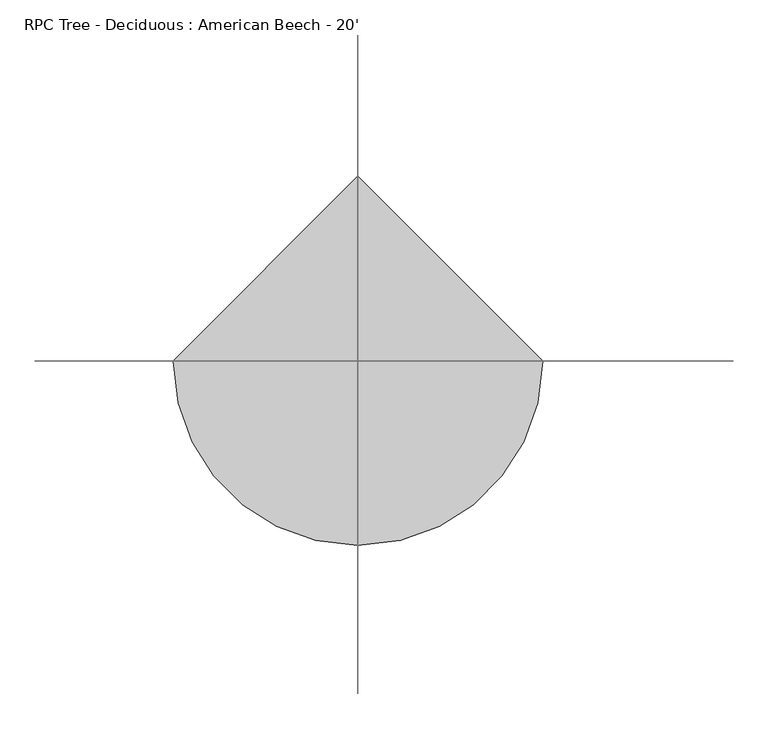
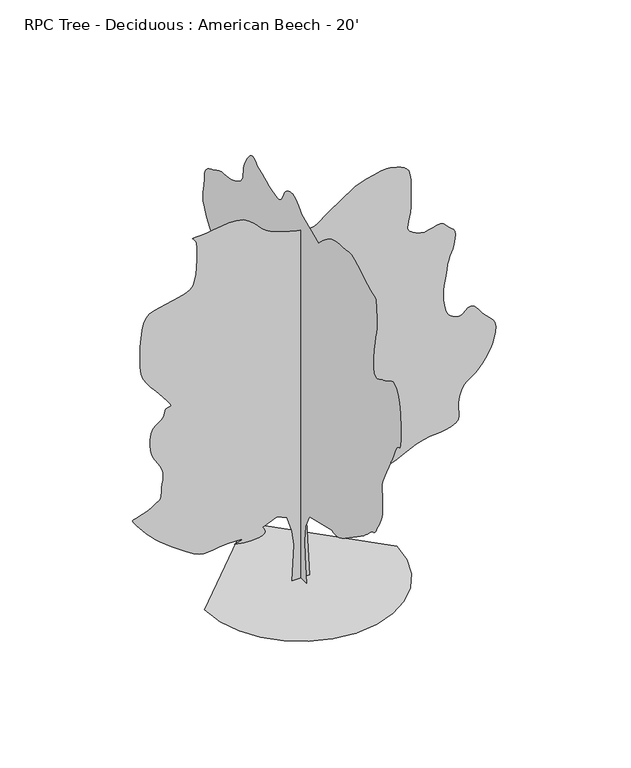
"""IFC4 building model written with IfcOpenShell, lengths in millimetres: geographic element geometry, RPC Tree - Deciduous : American Beech - 20'."""

import ifcopenshell
import ifcopenshell.guid

model = None  # the IFC model being written
_history = None  # IfcOwnerHistory: only IFC2X3 demands one
_inside = {}  # id of a spatial element -> (the spatial element, [elements in it])
_under = {}  # id of a project, library or spatial element -> (it, [spatial elements below it])
_declared = {}  # id of a project -> (the project, [libraries it declares])
_typed = {}  # id of a type object -> (the type object, [elements of that type])
_made_of = {}  # id of a material, layer set ... -> (it, [elements and type objects made of it])


def new_model(schema):
    """Start an empty IFC model of exactly this schema.

    Asked for "IFC4X3", IfcOpenShell would pick the latest addendum, in which some entities
    have other attributes; the version numbers below select the first issue.
    IFC2X3 requires an IfcOwnerHistory on every rooted entity: one is made here for all.
    """
    global model, _history
    if schema == "IFC4X3":
        model = ifcopenshell.file(schema_version=(4, 3, 0, 0))
    else:
        model = ifcopenshell.file(schema=schema)
    _inside.clear()
    _under.clear()
    _declared.clear()
    _typed.clear()
    _made_of.clear()
    _history = None
    if model.schema == "IFC2X3":
        org = make("IfcOrganization", Name="unknown")
        user = make(
            "IfcPersonAndOrganization",
            ThePerson=make("IfcPerson", FamilyName="unknown"),
            TheOrganization=org,
        )
        app = make(
            "IfcApplication",
            ApplicationDeveloper=org,
            Version="unknown",
            ApplicationFullName="unknown",
            ApplicationIdentifier="unknown",
        )
        _history = make(
            "IfcOwnerHistory",
            OwningUser=user,
            OwningApplication=app,
            ChangeAction="ADDED",
            CreationDate=0,
        )
    return model


def make(cls, **values):
    """One entity of the class cls with the attributes given. An attribute that is None is left unset."""
    return model.create_entity(
        cls, **{name: value for name, value in values.items() if value is not None}
    )


def rooted(cls, **values):
    """An entity with a GlobalId (a new one), such as an element, a storey or a relation."""
    return make(cls, GlobalId=ifcopenshell.guid.new(), OwnerHistory=_history, **values)


def si_unit(unit_type, name, prefix=None):
    """IfcSIUnit, for example si_unit("LENGTHUNIT", "METRE", prefix="MILLI")."""
    return make("IfcSIUnit", UnitType=unit_type, Prefix=prefix, Name=name)


def assignment(units):
    """IfcUnitAssignment: the units of a project."""
    return None if units is None else make("IfcUnitAssignment", Units=units)


def point(xyz):
    """IfcCartesianPoint."""
    return None if xyz is None else make("IfcCartesianPoint", Coordinates=xyz)


def direction(xyz):
    """IfcDirection."""
    return None if xyz is None else make("IfcDirection", DirectionRatios=xyz)


def frame(location, z_axis=None, x_axis=None):
    """IfcAxis2Placement3D, a coordinate frame: its origin and axes. An axis left out is left unset."""
    return make(
        "IfcAxis2Placement3D",
        Location=point(location),
        Axis=direction(z_axis),
        RefDirection=direction(x_axis),
    )


def origin():
    """The frame at (0, 0, 0) with its axes left unset."""
    return frame((0.0, 0.0, 0.0))


def place(relative_to, where):
    """IfcLocalPlacement: puts the frame where relative to a parent placement (None: the world)."""
    return make(
        "IfcLocalPlacement", PlacementRelTo=relative_to, RelativePlacement=where
    )


def context(
    kind, dimensions, precision=None, world=None, true_north=None, identifier=None
):
    """IfcGeometricRepresentationContext, for example the 3D "Model" context."""
    return make(
        "IfcGeometricRepresentationContext",
        ContextIdentifier=identifier,
        ContextType=kind,
        CoordinateSpaceDimension=dimensions,
        Precision=precision,
        WorldCoordinateSystem=world,
        TrueNorth=true_north,
    )


def project(units=None, contexts=None):
    """IfcProject with its units and contexts."""
    return rooted(
        "IfcProject",
        Name="project",
        RepresentationContexts=contexts,
        UnitsInContext=assignment(units),
    )


def spatial(cls, under=None, at=None, **own):
    """A site, building, storey or space (cls), placed at a placement, below another one or the project."""
    s = rooted(cls, ObjectPlacement=at, **own)
    if under is not None:
        _under.setdefault(under.id(), (under, []))[1].append(s)
    return s


def point_list(points):
    """IfcCartesianPointList2D or 3D."""
    cls = (
        "IfcCartesianPointList2D" if len(points[0]) == 2 else "IfcCartesianPointList3D"
    )
    return make(cls, CoordList=points)


def triangles(points, corners, closed=None, point_numbers=None):
    """IfcTriangulatedFaceSet: each triangle names its three corners, points numbered from 1."""
    return make(
        "IfcTriangulatedFaceSet",
        Coordinates=point_list(points),
        Closed=closed,
        CoordIndex=corners,
        PnIndex=point_numbers,
    )


def shape(context_of_items, identifier, shape_type, items):
    """IfcShapeRepresentation: the items that make up one representation, for example the "Body"."""
    return make(
        "IfcShapeRepresentation",
        ContextOfItems=context_of_items,
        RepresentationIdentifier=identifier,
        RepresentationType=shape_type,
        Items=items,
    )


def source(mapping_origin, context_of_items, identifier, shape_type, items):
    """IfcRepresentationMap: a shape defined once, which mapped items show again and again."""
    return make(
        "IfcRepresentationMap",
        MappingOrigin=mapping_origin,
        MappedRepresentation=shape(context_of_items, identifier, shape_type, items),
    )


def transform(
    local_origin,
    x_axis=None,
    y_axis=None,
    z_axis=None,
    scale=None,
    scale2=None,
    scale3=None,
    uniform=True,
):
    """IfcCartesianTransformationOperator3D, or its non-uniform kind. x_axis, y_axis, z_axis: its Axis1, 2, 3."""
    if uniform:
        return make(
            "IfcCartesianTransformationOperator3D",
            Axis1=direction(x_axis),
            Axis2=direction(y_axis),
            LocalOrigin=point(local_origin),
            Scale=scale,
            Axis3=direction(z_axis),
        )
    return make(
        "IfcCartesianTransformationOperator3DnonUniform",
        Axis1=direction(x_axis),
        Axis2=direction(y_axis),
        LocalOrigin=point(local_origin),
        Scale=scale,
        Axis3=direction(z_axis),
        Scale2=scale2,
        Scale3=scale3,
    )


def mapped(mapping_source, mapping_target):
    """IfcMappedItem: shows the shape of a source again, moved by a transform."""
    return make(
        "IfcMappedItem", MappingSource=mapping_source, MappingTarget=mapping_target
    )


def made_of(thing, what):
    """Note that an element or type object is made of a material, layer set ...; save() writes the relation."""
    if what is not None:
        _made_of.setdefault(what.id(), (what, []))[1].append(thing)
    return thing


def element(
    cls,
    number,
    at=None,
    inside=None,
    cuts=None,
    type_object=None,
    material=None,
    context=None,
    identifier="Body",
    shape_type=None,
    held_by="IfcProductDefinitionShape",
    body=None,
    shapes=None,
    **own,
):
    """One element of the class cls, such as IfcWall. Its Tag is "e" and its number.

    at: its placement. inside: the storey or other place that contains it. cuts: it is an
    opening in that element (IfcRelVoidsElement). A single representation is given by context,
    identifier, shape_type and body (its items); several are given by shapes. held_by: the class
    of the entity that holds the representations. save() writes the other relations.
    """
    e = rooted(cls, Tag="e%d" % number, ObjectPlacement=at, **own)
    if body is not None:
        shapes = [shape(context, identifier, shape_type, body)]
    if shapes is not None:
        e.Representation = make(held_by, Representations=shapes)
    if inside is not None:
        _inside.setdefault(inside.id(), (inside, []))[1].append(e)
    if cuts is not None:
        rooted(
            "IfcRelVoidsElement", RelatingBuildingElement=cuts, RelatedOpeningElement=e
        )
    if type_object is not None:
        _typed.setdefault(type_object.id(), (type_object, []))[1].append(e)
    return made_of(e, material)


def aggregate(whole, parts):
    """IfcRelAggregates: a whole, such as a stair, and the parts it consists of."""
    return rooted("IfcRelAggregates", RelatingObject=whole, RelatedObjects=parts)


def save(model, path):
    """Write the relations noted so far, then the file.

    IfcRelAggregates (storeys below a building ...), IfcRelContainedInSpatialStructure (elements
    in a storey), IfcRelDefinesByType, IfcRelAssociatesMaterial and IfcRelDeclares: one each for
    every whole, place, type object, material and project.
    """
    for whole, parts in _under.values():
        aggregate(whole, parts)
    for where, things in _inside.values():
        rooted(
            "IfcRelContainedInSpatialStructure",
            RelatedElements=things,
            RelatingStructure=where,
        )
    for kind, things in _typed.values():
        rooted("IfcRelDefinesByType", RelatedObjects=things, RelatingType=kind)
    for what, things in _made_of.values():
        rooted("IfcRelAssociatesMaterial", RelatedObjects=things, RelatingMaterial=what)
    for by, libraries in _declared.values():
        rooted("IfcRelDeclares", RelatingContext=by, RelatedDefinitions=libraries)
    model.write(path)


def rpc_tree_deciduous_american_beech_20_b3c041c8(model_context):
    return source(origin(), model_context, "Body", "Tessellation", [
        triangles([(0.0009889, 136.856581, 0.0), (0.0009889, -149.8547884, 0.0), (0.0009889, -111.6264895, 420.510052), (0.0009889, -102.0697236, 659.4353302), (0.0009889, -121.1832463, 898.3606447), (0.0009889, -235.8678885, 1118.172373), (0.0009889, -818.8458761, 1261.5275036), (0.0009889, -849.9431059, 1249.7139805), (0.0009889, -883.2933231, 1240.7427258), (0.0009889, -921.1596891, 1237.4533916), (0.0009889, -965.7976622, 1242.6934788), (0.0009889, -1019.4603024, 1259.3000233), (0.0009889, -1084.4081549, 1290.1152935), (0.0009889, -1162.8992941, 1337.984174), (0.0009889, -1478.2811337, 1557.7959023), (0.0009889, -1522.8632961, 1589.1420994), (0.0009889, -1566.942437, 1618.9819931), (0.0009889, -1611.1893002, 1649.3249084), (0.0009889, -1656.2718681, 1682.1772636), (0.0009889, -1702.8579781, 1719.5406807), (0.0009889, -1751.6183739, 1763.4243393), (0.0009889, -1803.2210381, 1815.834803), (0.0009889, -1847.9404015, 1858.0191467), (0.0009889, -1878.9512993, 1877.1351311), (0.0009889, -1901.2702858, 1884.0440117), (0.0009889, -1919.9112991, 1889.616782), (0.0009889, -1939.8884228, 1904.7196392), (0.0009889, -1966.2180656, 1940.2161644), (0.0009889, -2003.916782, 2006.9774963), (0.0009889, -2044.9607883, 2083.2080177), (0.0009889, -2078.313549, 2145.2324295), (0.0009889, -2104.4754696, 2201.0692829), (0.0009889, -2123.9521877, 2258.7475937), (0.0009889, -2137.244109, 2326.2862038), (0.0009889, -2144.8488773, 2411.7141289), (0.0009889, -2147.2746014, 2523.0550072), (0.0009889, -2142.5373905, 2624.8889076), (0.0009889, -2132.7863869, 2688.2873634), (0.0009889, -2124.7040314, 2730.9338882), (0.0009889, -2124.9835201, 2770.583503), (0.0009889, -2140.3072941, 2824.9394875), (0.0009889, -2177.3659332, 2911.7568626), (0.0009889, -2242.84464, 3048.6883301), (0.0009889, -2308.7119858, 3181.9621719), (0.0009889, -2348.5011269, 3259.3812836), (0.0009889, -2371.2366577, 3301.215358), (0.0009889, -2385.9484051, 3327.6567673), (0.0009889, -2401.6632889, 3358.9496246), (0.0009889, -2427.4088104, 3415.3121727), (0.0009889, -2472.2118896, 3516.9885246), (0.0009889, -2522.8114174, 3609.6476944), (0.0009889, -2561.0332123, 3645.1568642), (0.0009889, -2588.5669968, 3652.9040657), (0.0009889, -2607.0580193, 3662.3273277), (0.0009889, -2618.2087921, 3702.8402618), (0.0009889, -2623.669796, 3803.856189), (0.0009889, -2625.117382, 3994.8390083), (0.0009889, -2615.3639076, 4210.713913), (0.0009889, -2589.2271309, 4371.4450905), (0.0009889, -2551.406765, 4483.8402649), (0.0009889, -2506.5400269, 4554.7824463), (0.0009889, -2459.3391289, 4591.1043571), (0.0009889, -2414.4802391, 4599.6895889), (0.0009889, -2376.641851, 4587.3705734), (0.0009889, -2343.8477772, 4566.9491455), (0.0009889, -2310.8862717, 4546.8576393), (0.0009889, -2277.5893215, 4527.4521378), (0.0009889, -2243.7921112, 4509.0116936), (0.0009889, -2209.3243023, 4491.9426773), (0.0009889, -2174.0232594, 4476.5250137), (0.0009889, -2137.7164639, 4463.1392029), (0.0009889, -2096.4236355, 4443.6572525), (0.0009889, -2049.6139927, 4418.4858238), (0.0009889, -2002.3013283, 4400.6805153), (0.0009889, -1959.504958, 4403.2713455), (0.0009889, -1926.2359131, 4439.313913), (0.0009889, -1907.5110386, 4521.8132378), (0.0009889, -1908.3467434, 4663.8246277), (0.0009889, -1923.6450829, 4819.4253044), (0.0009889, -1942.954224, 4940.7356323), (0.0009889, -1963.266647, 5037.9669067), (0.0009889, -1981.572361, 5121.3298416), (0.0009889, -1994.8642822, 5201.0354416), (0.0009889, -2000.1296585, 5287.2429703), (0.0009889, -1994.3614059, 5390.1634323), (0.0009889, -1986.3653824, 5488.9190323), (0.0009889, -1983.048143, 5559.911792), (0.0009889, -1978.5625156, 5609.3407516), (0.0009889, -1967.0562412, 5643.3764648), (0.0009889, -1942.6748806, 5668.2429703), (0.0009889, -1899.5709709, 5690.0869858), (0.0009889, -1831.8926891, 5715.1063889), (0.0009889, -1748.4408062, 5751.9616974), (0.0009889, -1662.820015, 5800.5261749), (0.0009889, -1576.3582867, 5853.7903656), (0.0009889, -1490.4020508, 5904.6919098), (0.0009889, -1406.2848015, 5946.2207703), (0.0009889, -1325.3426491, 5971.3924896), (0.0009889, -1248.913884, 5973.1447083), (0.0009889, -1174.2403896, 5963.3406555), (0.0009889, -1098.5636135, 5956.711409), (0.0009889, -1023.222064, 5950.5641098), (0.0009889, -949.5518515, 5942.2588028), (0.0009889, -878.8914843, 5929.1264648), (0.0009889, -812.5771454, 5908.4509827), (0.0009889, -751.9472706, 5877.5644958), (0.0009889, -697.9494038, 5841.2678741), (0.0009889, -649.9687569, 5805.9618896), (0.0009889, -607.0045916, 5771.4942261), (0.0009889, -568.0511189, 5737.7119858), (0.0009889, -532.1075644, 5704.4128555), (0.0009889, -498.1706097, 5671.4433563), (0.0009889, -465.2369368, 5638.6523346), (0.0009889, -16.056217, 5829.7871796), (0.0009889, 22.8405617, 5872.4339951), (0.0009889, 61.6537222, 5913.023378), (0.0009889, 100.2998553, 5949.3961578), (0.0009889, 138.6950317, 5979.5204819), (0.0009889, 176.7559443, 6001.2883392), (0.0009889, 214.3990318, 6012.5911377), (0.0009889, 251.5404602, 6011.3720261), (0.0009889, 287.2056524, 6002.4312927), (0.0009889, 320.3628219, 5991.305809), (0.0009889, 350.8454089, 5977.0055191), (0.0009889, 378.4856913, 5958.5397858), (0.0009889, 403.1160919, 5934.892392), (0.0009889, 424.5689612, 5905.047702), (0.0009889, 442.6817001, 5868.0144974), (0.0009889, 459.9562634, 5826.9425858), (0.0009889, 480.2407084, 5787.547316), (0.0009889, 505.3740581, 5752.6727005), (0.0009889, 537.1926464, 5725.138916), (0.0009889, 577.5380399, 5707.7911377), (0.0009889, 628.2491524, 5703.5239563), (0.0009889, 691.1650068, 5715.1063889), (0.0009889, 759.6790661, 5736.9754028), (0.0009889, 826.1890326, 5761.3593796), (0.0009889, 891.0251186, 5787.8263687), (0.0009889, 954.5251671, 5815.9694183), (0.0009889, 1017.0218611, 5845.3577408), (0.0009889, 1078.8506453, 5875.5832214), (0.0009889, 1140.3440575, 5906.2412338), (0.0009889, 1169.0715191, 5932.3524307), (0.0009889, 1198.1316639, 5955.3649796), (0.0009889, 1227.8624073, 5972.2052307), (0.0009889, 1258.5938164, 5979.7489563), (0.0009889, 1290.6664227, 5974.9230881), (0.0009889, 1324.4078224, 5954.6539764), (0.0009889, 1360.1557858, 5915.7918137), (0.0009889, 1395.1799561, 5868.217392), (0.0009889, 1426.1908539, 5822.9544571), (0.0009889, 1452.6880737, 5778.8856354), (0.0009889, 1474.1715008, 5734.7912338), (0.0009889, 1490.1379681, 5689.5538788), (0.0009889, 1500.0845993, 5641.9538773), (0.0009889, 1503.510989, 5590.8494385), (0.0009889, 1507.2168674, 5539.3380478), (0.0009889, 1519.1142517, 5491.1793594), (0.0009889, 1540.3740005, 5446.1704788), (0.0009889, 1572.1672634, 5404.1846695), (0.0009889, 1615.6596668, 5365.0428726), (0.0009889, 1672.0274471, 5328.5689362), (0.0009889, 1742.4363762, 5294.5832199), (0.0009889, 1817.5288857, 5269.1836075), (0.0009889, 1887.9378147, 5255.1373718), (0.0009889, 1954.8363476, 5247.4407486), (0.0009889, 2019.3956337, 5241.0911362), (0.0009889, 2082.7839157, 5231.0580276), (0.0009889, 2146.1721977, 5212.3382401), (0.0009889, 2210.7313385, 5179.9024292), (0.0009889, 2276.3498623, 5145.3580261), (0.0009889, 2340.1267834, 5118.8404587), (0.0009889, 2399.0573433, 5093.1356323), (0.0009889, 2450.1315514, 5061.106192), (0.0009889, 2490.3372368, 5015.5136261), (0.0009889, 2516.667025, 4949.193837), (0.0009889, 2526.1132507, 4854.9597633), (0.0009889, 2532.46577, 4758.008123), (0.0009889, 2546.5044479, 4681.9348595), (0.0009889, 2560.7285797, 4617.2411339), (0.0009889, 2567.5865913, 4554.3760757), (0.0009889, 2559.5600464, 4483.8402649), (0.0009889, 2529.1232414, 4396.0578323), (0.0009889, 2468.7702393, 4281.5543564), (0.0009889, 2394.0992157, 4166.6192207), (0.0009889, 2326.6139454, 4078.2525215), (0.0009889, 2267.6553349, 4007.9707649), (0.0009889, 2218.5596397, 3947.1884285), (0.0009889, 2180.6679119, 3887.4223091), (0.0009889, 2155.3111748, 3820.1377533), (0.0009889, 2143.8328056, 3736.8001076), (0.0009889, 2149.4334812, 3646.0204742), (0.0009889, 2171.0820145, 3561.7686401), (0.0009889, 2203.7667927, 3483.5112076), (0.0009889, 2242.4687908, 3410.790937), (0.0009889, 2282.1714546, 3343.1000107), (0.0009889, 2317.8662235, 3279.9047401), (0.0009889, 2344.5311657, 3220.7225967), (0.0009889, 2370.3577869, 3180.6921913), (0.0009889, 2402.5396889, 3164.8934464), (0.0009889, 2434.5538685, 3157.7813805), (0.0009889, 2459.8827003, 3143.8113029), (0.0009889, 2472.0037628, 3107.4638123), (0.0009889, 2464.3963783, 3033.1433487), (0.0009889, 2430.5432121, 2905.3305107), (0.0009889, 2383.9011463, 2761.3378464), (0.0009889, 2340.6017544, 2643.9136185), (0.0009889, 2298.1379219, 2545.7425758), (0.0009889, 2254.0028252, 2459.415287), (0.0009889, 2205.6894951, 2377.6095245), (0.0009889, 2150.6857304, 2292.9614937), (0.0009889, 2086.4897942, 2198.1177189), (0.0009889, 2022.098085, 2102.5196297), (0.0009889, 1968.0723129, 2019.6267242), (0.0009889, 1924.2446102, 1948.102747), (0.0009889, 1890.4447838, 1886.6067913), (0.0009889, 1866.5103436, 1833.8078339), (0.0009889, 1852.2735672, 1788.3620613), (0.0009889, 1847.564407, 1748.9361248), (0.0009889, 1851.5776794, 1721.8800728), (0.0009889, 1860.940044, 1709.2029396), (0.0009889, 1871.6386642, 1703.0459026), (0.0009889, 1879.6624477, 1695.5504299), (0.0009889, 1881.0010288, 1678.8600243), (0.0009889, 1871.6386642, 1645.1186245), (0.0009889, 1847.564407, 1586.4675533), (0.0009889, 1827.5314728, 1524.5828133), (0.0009889, 1825.3850922, 1482.2587978), (0.0009889, 1829.7590984, 1453.3104195), (0.0009889, 1829.2865982, 1431.547649), (0.0009889, 1812.5961926, 1410.7907764), (0.0009889, 1768.3214241, 1384.8497726), (0.0009889, 1685.0958355, 1347.5421661), (0.0009889, 1594.399918, 1309.4244347), (0.0009889, 1528.281134, 1282.5080544), (0.0009889, 1476.2059696, 1262.7823689), (0.0009889, 1427.6412014, 1246.2316349), (0.0009889, 1372.05317, 1228.8453415), (0.0009889, 1298.9138844, 1206.6102161), (0.0009889, 1197.6871416, 1175.5154572), (0.0009889, 1096.069289, 1145.7009253), (0.0009889, 1022.5387482, 1127.7557997), (0.0009889, 967.7331545, 1118.3400227), (0.0009889, 922.2874546, 1114.10329), (0.0009889, 876.8442255, 1111.7080873), (0.0009889, 822.0360884, 1107.806654), (0.0009889, 748.5055475, 1099.0588594), (0.0009889, 662.4935011, 1085.0990284), (0.0009889, 576.4788749, 1068.1292793), (0.0009889, 490.4667558, 1048.6551046), (0.0009889, 404.4521296, 1027.1717503), (0.0009889, 318.4400468, 1004.1847086), (0.0009889, 232.4266923, 980.1943851), (0.0009889, 146.4133378, 955.7037289), (136.1842383, 0.0003154, 0.014068), (-131.4120823, 0.0003154, 0.014068), (-102.7410489, 0.0002819, 563.8778998), (-131.4120823, 0.0002692, 793.2477293), (-207.8684348, 0.0002549, 1032.1729712), (-360.7819027, 0.0002501, 1108.6296415), (-580.5936673, 0.0002549, 1013.0594576), (-562.704425, 0.0002564, 988.5662579), (-548.0765751, 0.000258, 964.5784779), (-539.9688578, 0.0002596, 941.5914362), (-541.6401947, 0.0002612, 920.1080818), (-556.3518694, 0.0002628, 900.6313637), (-587.3627672, 0.0002628, 883.6641581), (-637.9342443, 0.0002644, 869.704327), (-697.421093, 0.0002644, 860.4815615), (-753.4001616, 0.0002644, 856.775683), (-806.4506298, 0.0002644, 857.667271), (-857.1617786, 0.0002644, 862.2366869), (-906.117802, 0.0002644, 869.5645826), (-953.9028214, 0.0002628, 878.731465), (-1001.1011759, 0.0002628, 888.8178406), (-953.2881786, 0.0002628, 900.9945683), (-913.501581, 0.0002612, 912.5008427), (-889.7601522, 0.0002612, 922.6710068), (-890.0954515, 0.0002596, 930.8345346), (-922.5287189, 0.0002596, 936.3235165), (-995.0838833, 0.0002596, 938.4698244), (-1115.7848007, 0.0002596, 936.6028599), (-1242.9524746, 0.0002612, 927.8271601), (-1337.3542706, 0.0002612, 914.3677345), (-1410.6891838, 0.0002612, 903.2500992), (-1474.6617325, 0.0002612, 901.4949738), (-1540.9759987, 0.0002612, 916.12286), (-1621.3340298, 0.0002596, 954.1568756), (-1727.4351116, 0.0002549, 1022.614979), (-1845.0726986, 0.0002501, 1105.8432564), (-1952.34711, 0.0002453, 1184.0549795), (-2049.4209812, 0.0002405, 1258.0858532), (-2136.46436, 0.0002373, 1328.7765965), (-2213.6472942, 0.0002326, 1396.9554291), (-2281.1300938, 0.0002278, 1463.4653229), (-2339.0852772, 0.0002246, 1529.1396572), (-2391.8031349, 0.0002214, 1592.6651402), (-2441.3431343, 0.0002166, 1651.1791557), (-2484.5309052, 0.0002134, 1703.170459), (-2518.1884438, 0.0002118, 1747.1378334), (-2539.1409439, 0.0002103, 1781.577737), (-2544.218541, 0.0002087, 1804.9838665), (-2530.2254997, 0.0002071, 1815.8500637), (-2498.742247, 0.0002071, 1822.7308937), (-2456.2227493, 0.0002071, 1834.628278), (-2406.8475655, 0.0002055, 1850.7065117), (-2354.8003063, 0.0002039, 1870.1272739), (-2304.2568798, 0.0002023, 1892.0551506), (-2259.3978447, 0.0002023, 1915.6542915), (-2224.401725, 0.0002007, 1940.091608), (-2196.9849392, 0.0001991, 1958.6464348), (-2172.4078056, 0.0001991, 1969.1798035), (-2151.1759621, 0.0001975, 1977.7066086), (-2133.7896687, 0.0001975, 1990.2439247), (-2120.7518017, 0.0001959, 2012.8144947), (-2112.5602959, 0.0001927, 2051.4326317), (-2109.7180275, 0.0001895, 2112.118317), (-2105.7607109, 0.0001864, 2181.0514641), (-2096.7894562, 0.0001816, 2242.2935108), (-2087.1476028, 0.0001784, 2298.6891964), (-2081.1861935, 0.0001752, 2353.0781731), (-2083.2487129, 0.000172, 2408.3028545), (-2097.6809715, 0.0001688, 2467.2028931), (-2128.8315411, 0.0001641, 2532.6259346), (-2168.3971493, 0.0001609, 2596.7202782), (-2204.2849297, 0.0001577, 2653.2860115), (-2235.1560104, 0.0001545, 2707.6675758), (-2259.6771881, 0.0001513, 2765.2239464), (-2276.5047947, 0.0001465, 2831.3149704), (-2284.3076614, 0.0001418, 2911.2740433), (-2281.7447365, 0.000137, 3010.4865921), (-2264.5514545, 0.0001306, 3102.7902603), (-2233.1494469, 0.0001274, 3164.9948936), (-2193.2231049, 0.0001242, 3206.8286774), (-2150.4520237, 0.0001226, 3237.9439293), (-2110.525827, 0.0001211, 3268.0682533), (-2079.123674, 0.0001179, 3306.8795471), (-2061.9330082, 0.0001147, 3364.0804161), (-2043.9599773, 0.0001131, 3413.0262657), (-2014.1200836, 0.0001115, 3431.3396828), (-1983.9422745, 0.0001115, 3435.3019409), (-1964.9684326, 0.0001099, 3441.0931572), (-1968.7301216, 0.0001099, 3464.9437363), (-2006.7641373, 0.0001051, 3523.0843735), (-2090.6020432, 9.88e-05, 3631.6948952), (-2191.4121689, 9.24e-05, 3753.7165169), (-2273.3296978, 8.6e-05, 3849.6778107), (-2337.3582024, 8.12e-05, 3932.1009773), (-2384.5031445, 7.65e-05, 4013.5079269), (-2415.7654804, 7.17e-05, 4106.47202), (-2432.1484921, 6.37e-05, 4223.4898773), (-2434.6554611, 5.42e-05, 4377.1345688), (-2429.5297565, 4.46e-05, 4541.5998207), (-2420.5585018, 3.66e-05, 4683.0016548), (-2405.0643894, 3.03e-05, 4801.6705742), (-2380.3781055, 2.39e-05, 4897.9365005), (-2343.822488, 1.91e-05, 4972.1558075), (-2292.720084, 1.59e-05, 5024.6066757), (-2224.401725, 1.43e-05, 5055.6710587), (-2138.4149677, 1.27e-05, 5074.7972168), (-2040.8941761, 1.27e-05, 5092.7292618), (-1939.0274288, 1.11e-05, 5111.8554199), (-1840.0028046, 9.6e-06, 5134.487178), (-1751.0088181, 8e-06, 5162.9604401), (-1679.2334026, 6.4e-06, 5199.612854), (-1631.8649277, 3.2e-06, 5246.8314835), (-1604.1128426, -1.6e-06, 5316.4272354), (-1585.3905842, -6.4e-06, 5411.6010773), (-1574.1890877, -1.27e-05, 5521.6594757), (-1569.0075726, -2.07e-05, 5635.9088974), (-1568.336974, -2.71e-05, 5743.6302292), (-1570.6788368, -3.19e-05, 5834.1305191), (-1574.524387, -3.5e-05, 5896.690654), (-1585.918895, -3.82e-05, 5936.1626633), (-1606.0102558, -3.98e-05, 5965.4230865), (-1625.9315689, -4.14e-05, 5985.9718323), (-1636.825526, -4.14e-05, 5999.3576431), (-1629.8329296, -4.3e-05, 6007.0286865), (-1596.0890591, -4.3e-05, 6010.559285), (-1526.7393677, -4.3e-05, 6011.3976059), (-1428.7715103, -4.3e-05, 6017.8233765), (-1318.7690678, -4.46e-05, 6032.4538788), (-1202.2439129, -4.46e-05, 6048.2529144), (-1084.7180197, -4.46e-05, 6058.184285), (-971.7057318, -4.46e-05, 6055.263533), (-868.7238636, -4.46e-05, 6032.4538788), (-781.2893749, -4.14e-05, 5982.7208679), (-714.8937183, -3.66e-05, 5922.6245361), (-665.5465851, -3.34e-05, 5871.6974121), (-624.5610781, -3.19e-05, 5827.4756927), (-583.2403444, -2.87e-05, 5787.445578), (-532.8924365, -2.71e-05, 5749.0915237), (-464.8228995, -2.39e-05, 5709.8735687), (-370.3373878, -2.23e-05, 5667.3284912), (-260.8632923, -1.91e-05, 5627.3745346), (-155.7366604, -1.75e-05, 5596.9449966), (-58.1322665, -1.59e-05, 5575.0504028), (28.7726351, -1.59e-05, 5560.6739548), (101.8020074, -1.59e-05, 5552.8255966), (157.7788323, -1.43e-05, 5550.4629501), (193.5270681, -1.59e-05, 5552.6477005), (219.2725352, -1.59e-05, 5560.6233765), (247.3583572, -1.59e-05, 5575.4311935), (277.7847885, -1.75e-05, 5595.7770447), (310.5508118, -1.91e-05, 5620.2877579), (345.6587342, -2.07e-05, 5647.6692261), (383.1059761, -2.23e-05, 5676.5232788), (422.8950809, -2.39e-05, 5705.555809), (805.1781057, -3.98e-05, 5963.5947098), (830.3647951, -3.98e-05, 5972.992392), (896.679134, -4.14e-05, 5996.5892075), (990.2426817, -4.3e-05, 6027.5518524), (1097.1817938, -4.62e-05, 6058.9970261), (1203.6180296, -4.62e-05, 6084.1175858), (1295.67789, -4.78e-05, 6096.0046509), (1359.4853325, -4.78e-05, 6087.8516602), (1407.4912685, -4.62e-05, 6070.6556168), (1459.1777939, -4.46e-05, 6056.8128571), (1511.1996185, -4.46e-05, 6041.4457718), (1560.2089817, -4.3e-05, 6019.7540726), (1602.8682964, -4.14e-05, 5986.835733), (1635.8299473, -3.82e-05, 5937.8898834), (1655.7537312, -3.34e-05, 5868.0394958), (1665.3091072, -2.87e-05, 5789.7820633), (1670.1859898, -2.55e-05, 5717.2399796), (1671.5500053, -2.07e-05, 5647.8471222), (1670.5746288, -1.75e-05, 5579.1396881), (1668.4282482, -1.27e-05, 5508.6038773), (1666.2844837, -8e-06, 5433.699147), (1665.3091072, -3.2e-06, 5351.9622757), (1660.2367424, 1.6e-06, 5270.5806152), (1648.1463467, 6.4e-06, 5198.4187408), (1633.7114719, 9.6e-06, 5135.2743393), (1621.6186054, 1.27e-05, 5081.0200928), (1616.5487114, 1.59e-05, 5035.4269455), (1623.1807194, 1.75e-05, 4998.368161), (1646.1955936, 1.91e-05, 4969.6664246), (1678.4054008, 2.07e-05, 4946.8317719), (1709.6119263, 2.23e-05, 4927.324823), (1739.9826015, 2.23e-05, 4910.992099), (1769.6829689, 2.39e-05, 4897.6824463), (1798.8852562, 2.39e-05, 4887.1923889), (1827.7499187, 2.55e-05, 4879.3946091), (1856.4493298, 2.55e-05, 4874.0862122), (1893.0609032, 2.55e-05, 4877.1087021), (1942.2125542, 2.39e-05, 4889.9864044), (1998.8851124, 2.39e-05, 4906.1918106), (2058.0671104, 2.23e-05, 4919.2474091), (2114.7396687, 2.23e-05, 4922.5745316), (2163.8911743, 2.39e-05, 4909.6968292), (2200.5028931, 2.55e-05, 4874.0862122), (2230.4850746, 2.71e-05, 4834.208123), (2261.3003448, 2.87e-05, 4807.6649757), (2290.2766285, 3.03e-05, 4786.8368866), (2314.7419956, 3.19e-05, 4763.9769447), (2332.0165226, 3.34e-05, 4731.4396866), (2339.4282795, 3.66e-05, 4681.5031998), (2334.3025749, 4.14e-05, 4606.4970222), (2319.8956055, 4.62e-05, 4526.9440292), (2302.1485783, 4.94e-05, 4463.951944), (2282.3925167, 5.26e-05, 4410.6627548), (2261.9683273, 5.57e-05, 4360.1928703), (2242.2147366, 5.89e-05, 4305.7098587), (2224.4652386, 6.37e-05, 4240.3809975), (2210.0608852, 6.85e-05, 4157.3229858), (2196.9087811, 7.33e-05, 4068.4481781), (2183.2562714, 7.8e-05, 3988.0827347), (2170.9397266, 8.28e-05, 3913.0762665), (2161.8007496, 8.76e-05, 3840.2289688), (2157.6783268, 9.08e-05, 3766.3913246), (2160.4088287, 9.56e-05, 3688.3876556), (2171.831242, 0.0001003, 3603.0181572), (2189.9719952, 0.0001051, 3525.0147789), (2211.6203831, 0.0001083, 3468.2711494), (2236.7791672, 0.0001115, 3428.240744), (2265.4506729, 0.0001131, 3400.402327), (2297.6324295, 0.0001147, 3380.2602425), (2333.3271984, 0.0001147, 3363.2673843), (2372.5296021, 0.0001163, 3344.9795471), (2412.5675652, 0.0001163, 3342.4901642), (2451.7724396, 0.0001147, 3366.0869797), (2491.642971, 0.0001131, 3400.8848557), (2533.6901138, 0.0001115, 3432.0253967), (2579.4227875, 0.0001099, 3444.5728867), (2630.3246223, 0.0001115, 3423.7195084), (2687.906282, 0.0001163, 3354.5298363), (2749.8568611, 0.0001211, 3269.9730789), (2810.1313797, 0.0001242, 3206.9557045), (2864.6905495, 0.0001274, 3156.6637161), (2909.5976921, 0.0001306, 3110.2325386), (2940.7635223, 0.0001338, 3058.7720169), (2954.2254913, 0.000137, 2993.4178665), (2945.9451828, 0.0001434, 2905.3557999), (2924.1520363, 0.0001481, 2810.6139084), (2899.209082, 0.0001529, 2729.079641), (2870.2277115, 0.0001577, 2657.6040619), (2836.3948929, 0.0001609, 2592.9612053), (2796.8723053, 0.0001641, 2531.9858574), (2750.8474983, 0.0001688, 2471.5235596), (2697.4568619, 0.000172, 2408.3842449), (2642.4404526, 0.0001752, 2354.2186558), (2591.9196991, 0.0001784, 2316.7713776), (2545.7425758, 0.00018, 2287.0127289), (2503.7637428, 0.0001816, 2255.9181152), (2465.7858284, 0.0001832, 2214.4575645), (2431.6531734, 0.000188, 2153.606773), (2401.2011078, 0.0001927, 2064.3332977), (2384.7901909, 0.0001991, 1965.7532684), (2385.7654221, 0.0002039, 1881.8849865), (2393.4261463, 0.0002071, 1811.0570423), (2397.0760689, 0.0002118, 1751.5981716), (2386.0143894, 0.000215, 1701.8343487), (2349.5424877, 0.0002166, 1660.0945999), (2276.9594181, 0.0002182, 1624.7096958), (2189.7484623, 0.0002198, 1601.1638947), (2111.7322941, 0.0002214, 1590.8261536), (2035.7202187, 0.0002214, 1585.8401207), (1954.5264828, 0.0002214, 1578.3445026), (1860.9630077, 0.000223, 1560.4858543), (1747.8389534, 0.0002246, 1524.4025917), (1607.9660957, 0.0002294, 1462.2385082), (1455.667543, 0.0002326, 1390.7425816), (1311.7282185, 0.0002357, 1331.4512878), (1178.6524023, 0.0002389, 1283.6941738), (1058.9547667, 0.0002421, 1246.8031116), (955.1372663, 0.0002437, 1220.1102642), (869.7094139, 0.0002437, 1202.9449602), (805.1781057, 0.0002453, 1194.641688), (403.7815673, 0.0002453, 1185.0862392), (107.513205, 0.0002485, 1137.3011473), (88.3996914, 0.0002628, 879.2597757), (-1453.7574852, 0.0, 0.0120292), (-1415.3246567, -333.1060121, 0.0120292), (-1305.8708725, -639.0085974, 0.0120292), (-1134.1566444, -908.9473532, 0.0120292), (-908.9473532, -1134.1566444, 0.0120292), (-639.0085974, -1305.8708725, 0.0120292), (-333.1060121, -1415.3246567, 0.0120292), (6.35e-05, -1453.7574852, 0.0120292), (333.1060121, -1415.3246567, 0.0120292), (639.0085974, -1305.8708725, 0.0120292), (908.9473532, -1134.1566444, 0.0120292), (1134.1566444, -908.9473532, 0.0120292), (1305.8708725, -639.0085974, 0.0120292), (1415.3246567, -333.1060121, 0.0120292), (1453.7574852, 0.0001274, 0.0120292), (-0.0001906, 1453.7574852, 0.0120292)], [[1, 2, 3], [254, 1, 3], [254, 3, 4], [254, 4, 5], [254, 5, 6], [53, 54, 55], [52, 53, 55], [201, 202, 203], [201, 203, 204], [200, 201, 204], [222, 223, 224], [52, 55, 56], [200, 204, 205], [199, 200, 205], [253, 254, 6], [221, 222, 224], [221, 224, 225], [229, 230, 231], [229, 231, 232], [228, 229, 232], [228, 232, 233], [227, 228, 233], [252, 253, 6], [221, 225, 226], [220, 221, 226], [199, 205, 206], [198, 199, 206], [62, 63, 64], [61, 62, 64], [61, 64, 65], [60, 61, 65], [60, 65, 66], [59, 60, 66], [59, 66, 67], [59, 67, 68], [58, 59, 68], [58, 68, 69], [58, 69, 70], [57, 58, 70], [57, 70, 71], [57, 71, 72], [57, 72, 73], [57, 73, 74], [56, 57, 74], [52, 56, 74], [51, 52, 74], [50, 51, 74], [50, 74, 75], [49, 50, 75], [48, 49, 75], [47, 48, 75], [46, 47, 75], [45, 46, 75], [44, 45, 75], [43, 44, 75], [42, 43, 75], [42, 75, 76], [41, 42, 76], [227, 233, 234], [226, 227, 234], [220, 226, 234], [219, 220, 234], [219, 234, 235], [219, 235, 236], [219, 236, 237], [218, 219, 237], [218, 237, 238], [218, 238, 239], [218, 239, 240], [217, 218, 240], [217, 240, 241], [217, 241, 242], [217, 242, 243], [217, 243, 244], [217, 244, 245], [217, 245, 246], [216, 217, 246], [216, 246, 247], [215, 216, 247], [215, 247, 248], [251, 252, 6], [88, 89, 90], [88, 90, 91], [87, 88, 91], [87, 91, 92], [86, 87, 92], [86, 92, 93], [85, 86, 93], [84, 85, 93], [84, 93, 94], [83, 84, 94], [82, 83, 94], [81, 82, 94], [81, 94, 95], [80, 81, 95], [80, 95, 96], [80, 96, 97], [80, 97, 98], [80, 98, 99], [80, 99, 100], [80, 100, 101], [80, 101, 102], [80, 102, 103], [80, 103, 104], [80, 104, 105], [80, 105, 106], [80, 106, 107], [80, 107, 108], [80, 108, 109], [80, 109, 110], [80, 110, 111], [80, 111, 112], [79, 80, 112], [79, 112, 113], [78, 79, 113], [77, 78, 113], [76, 77, 113], [41, 76, 113], [40, 41, 113], [40, 113, 114], [39, 40, 114], [198, 206, 207], [197, 198, 207], [196, 197, 207], [196, 207, 208], [195, 196, 208], [195, 208, 209], [195, 209, 210], [195, 210, 211], [194, 195, 211], [194, 211, 212], [194, 212, 213], [193, 194, 213], [193, 213, 214], [214, 215, 248], [193, 214, 248], [193, 248, 249], [192, 193, 249], [192, 249, 250], [192, 250, 251], [192, 251, 6], [192, 6, 7], [191, 192, 7], [190, 191, 7], [189, 190, 7], [38, 39, 114], [37, 38, 114], [36, 37, 114], [35, 36, 114], [34, 35, 114], [33, 34, 114], [32, 33, 114], [31, 32, 114], [30, 31, 114], [29, 30, 114], [28, 29, 114], [27, 28, 114], [26, 27, 114], [25, 26, 114], [24, 25, 114], [23, 24, 114], [22, 23, 114], [21, 22, 114], [20, 21, 114], [19, 20, 114], [18, 19, 114], [17, 18, 114], [16, 17, 114], [15, 16, 114], [14, 15, 114], [13, 14, 114], [12, 13, 114], [11, 12, 114], [10, 11, 114], [9, 10, 114], [8, 9, 114], [7, 8, 114], [189, 7, 114], [188, 189, 114], [188, 114, 115], [188, 115, 116], [188, 116, 117], [188, 117, 118], [188, 118, 119], [188, 119, 120], [188, 120, 121], [146, 147, 148], [145, 146, 148], [144, 145, 148], [144, 148, 149], [143, 144, 149], [143, 149, 150], [142, 143, 150], [142, 150, 151], [142, 151, 152], [141, 142, 152], [141, 152, 153], [141, 153, 154], [141, 154, 155], [141, 155, 156], [140, 141, 156], [140, 156, 157], [139, 140, 157], [138, 139, 157], [138, 157, 158], [137, 138, 158], [137, 158, 159], [136, 137, 159], [135, 136, 159], [135, 159, 160], [134, 135, 160], [134, 160, 161], [174, 175, 176], [173, 174, 176], [173, 176, 177], [172, 173, 177], [171, 172, 177], [171, 177, 178], [170, 171, 178], [170, 178, 179], [169, 170, 179], [168, 169, 179], [167, 168, 179], [166, 167, 179], [165, 166, 179], [165, 179, 180], [165, 180, 181], [165, 181, 182], [165, 182, 183], [165, 183, 184], [165, 184, 185], [165, 185, 186], [165, 186, 187], [164, 165, 187], [164, 187, 188], [163, 164, 188], [162, 163, 188], [161, 162, 188], [134, 161, 188], [133, 134, 188], [132, 133, 188], [125, 126, 127], [124, 125, 127], [124, 127, 128], [123, 124, 128], [122, 123, 128], [121, 122, 128], [121, 128, 129], [121, 129, 130], [121, 130, 131], [188, 121, 131], [132, 188, 131], [274, 275, 276], [531, 255, 256], [531, 256, 257], [531, 257, 258], [531, 258, 259], [530, 531, 259], [376, 377, 378], [376, 378, 379], [375, 376, 379], [273, 274, 276], [273, 276, 277], [375, 379, 380], [374, 375, 380], [273, 277, 278], [272, 273, 278], [301, 302, 303], [301, 303, 304], [300, 301, 304], [300, 304, 305], [299, 300, 305], [299, 305, 306], [298, 299, 306], [298, 306, 307], [297, 298, 307], [297, 307, 308], [271, 272, 278], [296, 297, 308], [296, 308, 309], [373, 374, 380], [373, 380, 381], [372, 373, 381], [295, 296, 309], [295, 309, 310], [294, 295, 310], [294, 310, 311], [294, 311, 312], [294, 312, 313], [293, 294, 313], [293, 313, 314], [292, 293, 314], [271, 278, 279], [291, 292, 314], [530, 259, 260], [372, 381, 382], [371, 372, 382], [291, 314, 315], [290, 291, 315], [371, 382, 383], [370, 371, 383], [370, 383, 384], [369, 370, 384], [369, 384, 385], [369, 385, 386], [369, 386, 387], [369, 387, 388], [369, 388, 389], [369, 389, 390], [368, 369, 390], [368, 390, 391], [367, 368, 391], [367, 391, 392], [367, 392, 393], [366, 367, 393], [366, 393, 394], [270, 271, 279], [366, 394, 395], [338, 339, 340], [338, 340, 341], [289, 290, 315], [483, 484, 485], [483, 485, 486], [482, 483, 486], [481, 482, 486], [481, 486, 487], [480, 481, 487], [288, 289, 315], [287, 288, 315], [286, 287, 315], [285, 286, 315], [284, 285, 315], [283, 284, 315], [282, 283, 315], [282, 315, 316], [281, 282, 316], [281, 316, 317], [281, 317, 318], [281, 318, 319], [281, 319, 320], [280, 281, 320], [280, 320, 321], [279, 280, 321], [279, 321, 322], [480, 487, 488], [264, 265, 266], [263, 264, 266], [263, 266, 267], [262, 263, 267], [262, 267, 268], [261, 262, 268], [261, 268, 269], [261, 269, 270], [261, 270, 279], [261, 279, 322], [260, 261, 322], [530, 260, 322], [530, 322, 323], [529, 530, 323], [529, 323, 324], [366, 395, 396], [365, 366, 396], [337, 338, 341], [337, 341, 342], [529, 324, 325], [528, 529, 325], [527, 528, 325], [526, 527, 325], [525, 526, 325], [524, 525, 325], [523, 524, 325], [522, 523, 325], [521, 522, 325], [521, 325, 326], [521, 326, 327], [521, 327, 328], [521, 328, 329], [521, 329, 330], [521, 330, 331], [521, 331, 332], [521, 332, 333], [521, 333, 334], [521, 334, 335], [521, 335, 336], [521, 336, 337], [521, 337, 342], [520, 521, 342], [520, 342, 343], [519, 520, 343], [518, 519, 343], [518, 343, 344], [517, 518, 344], [449, 450, 451], [448, 449, 451], [448, 451, 452], [447, 448, 452], [446, 447, 452], [446, 452, 453], [516, 517, 344], [515, 516, 344], [514, 515, 344], [513, 514, 344], [512, 513, 344], [511, 512, 344], [510, 511, 344], [509, 510, 344], [508, 509, 344], [507, 508, 344], [506, 507, 344], [505, 506, 344], [504, 505, 344], [503, 504, 344], [502, 503, 344], [501, 502, 344], [500, 501, 344], [499, 500, 344], [498, 499, 344], [497, 498, 344], [496, 497, 344], [495, 496, 344], [494, 495, 344], [493, 494, 344], [492, 493, 344], [491, 492, 344], [490, 491, 344], [489, 490, 344], [488, 489, 344], [480, 488, 344], [479, 480, 344], [478, 479, 344], [477, 478, 344], [476, 477, 344], [475, 476, 344], [474, 475, 344], [473, 474, 344], [472, 473, 344], [471, 472, 344], [470, 471, 344], [469, 470, 344], [468, 469, 344], [467, 468, 344], [466, 467, 344], [465, 466, 344], [464, 465, 344], [463, 464, 344], [463, 344, 345], [462, 463, 345], [462, 345, 346], [461, 462, 346], [460, 461, 346], [459, 460, 346], [458, 459, 346], [457, 458, 346], [456, 457, 346], [455, 456, 346], [454, 455, 346], [453, 454, 346], [446, 453, 346], [445, 446, 346], [444, 445, 346], [443, 444, 346], [442, 443, 346], [441, 442, 346], [440, 441, 346], [439, 440, 346], [438, 439, 346], [437, 438, 346], [436, 437, 346], [435, 436, 346], [435, 346, 347], [435, 347, 348], [435, 348, 349], [435, 349, 350], [435, 350, 351], [435, 351, 352], [435, 352, 353], [435, 353, 354], [435, 354, 355], [435, 355, 356], [435, 356, 357], [435, 357, 358], [435, 358, 359], [435, 359, 360], [435, 360, 361], [435, 361, 362], [435, 362, 363], [435, 363, 364], [435, 364, 365], [435, 365, 396], [435, 396, 397], [435, 397, 398], [435, 398, 399], [435, 399, 400], [435, 400, 401], [435, 401, 402], [435, 402, 403], [435, 403, 404], [435, 404, 405], [435, 405, 406], [435, 406, 407], [435, 407, 408], [435, 408, 409], [434, 435, 409], [433, 434, 409], [432, 433, 409], [431, 432, 409], [430, 431, 409], [429, 430, 409], [429, 409, 410], [429, 410, 411], [429, 411, 412], [428, 429, 412], [428, 412, 413], [427, 428, 413], [426, 427, 413], [426, 413, 414], [425, 426, 414], [425, 414, 415], [425, 415, 416], [425, 416, 417], [424, 425, 417], [424, 417, 418], [423, 424, 418], [423, 418, 419], [422, 423, 419], [422, 419, 420], [421, 422, 420], [546, 547, 532], [545, 546, 532], [545, 532, 533], [544, 545, 533], [544, 533, 534], [544, 534, 535], [543, 544, 535], [542, 543, 535], [542, 535, 536], [542, 536, 537], [542, 537, 538], [542, 538, 539], [542, 539, 540], [542, 540, 541]], closed=False),
    ])


if __name__ == "__main__":
    model = new_model("IFC4")
    model_context = context("Model", 3, world=origin())
    ifc_project = project(units=[si_unit("LENGTHUNIT", "METRE", prefix="MILLI")], contexts=[model_context])
    site = spatial("IfcSite", under=ifc_project)
    building = spatial("IfcBuilding", under=site)
    placement = place(None, origin())
    rpc_tree_deciduous_american_beech_20_shape = rpc_tree_deciduous_american_beech_20_b3c041c8(model_context)
    element("IfcGeographicElement", 1, ObjectType="RPC Tree - Deciduous : American Beech - 20'", at=placement, inside=building, context=model_context, shape_type="MappedRepresentation", body=[
        mapped(rpc_tree_deciduous_american_beech_20_shape, transform((0.0, 0.0, 0.0), x_axis=(1.0, 0.0, 0.0), y_axis=(0.0, 1.0, 0.0), z_axis=(0.0, 0.0, 1.0))),
    ])
    save(model, "model.ifc")

# Revit data of these elements
# Type "RPC Tree - Deciduous : American Beech - 20'"
#   built-in parameter 1005198 = "{2, 15},{39, RPC-16-G1GQ-43Q0-7NP3-0000-ST1L-LVER-AU},{1, 0},{1, 0},{2, 13},{1, 8},{5, Color},{1, 0},{1, 0},{3, 0.8},{3, 0.8},{3, 0.8},{1, 8},{7, BBoxMin},{1, 0},{1, 0},{1, 0},{1, 0},{1, 0},{1, 8},{7, BBoxMax},{1, 0},{1, 0},{1, 0},{1, 0},{1, 0},{2, 11},{9, RPCTypeId},{1, 0},{1, 0},{39, RPC-16-G1GQ-43Q0-7NP3-0000-ST1L-LVER-AU},{1, 6},{14, RPCPlantHeight},{1, 0},{1, 0},{2, 20},{2, 11},{7, keyword},{1, 0},{1, 0},{34, :RPCs:Trees [General]:Geometry:RPC},{2, 11},{8, category},{1, 0},{1, 0},{15, Trees [General]},{2, 11},{12, LocalizedUID},{1, 0},{1, 0},{14, American Beech},{2, 14},{6, Height},{1, 0},{1, 0},{2, 20},{1, 2},{16, Cast Reflections},{1, 0},{1, 0},{1, 0},{1, 2},{12, Cast Shadows},{1, 0},{1, 0},{1, 1},{1, 2},{9, Lock View},{1, 0},{1, 0},{1, 0},{1, 4},{5, ViewC},{1, 0},{1, 0},{1, 0},{21, assetlibrary_base.fbx},{1, 5},"
#   built-in parameter 1005195 = "RPC-16-G1GQ-43Q0-7NP3-0000-ST1L-LVER-AU"
#   Type Comments = "American Beech"
#   Assembly Code = "G2050500"
#   Height = 20.00 ft
#   Default Elevation = 0
